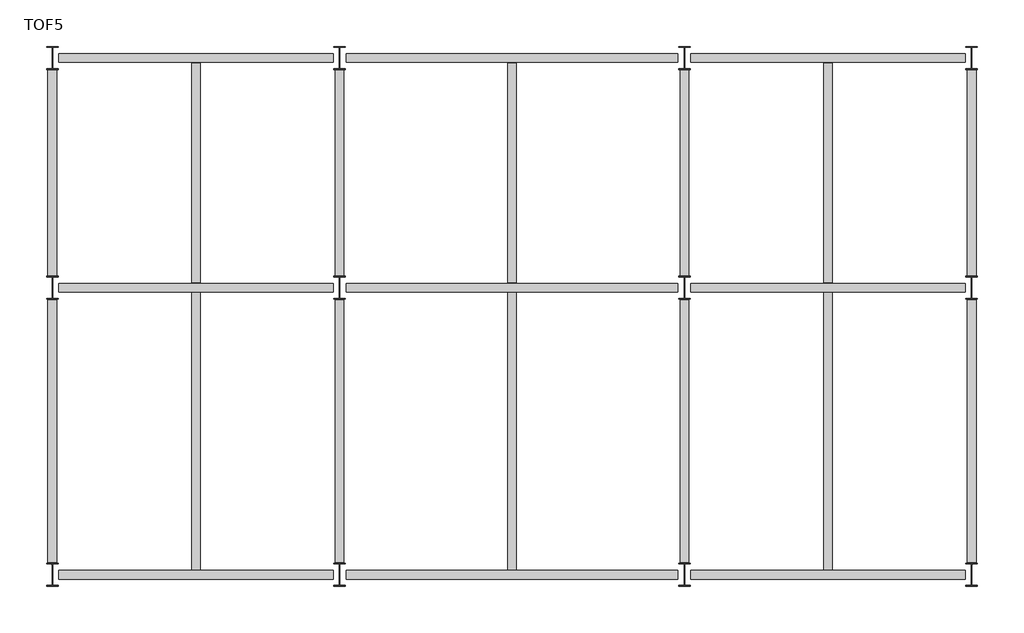
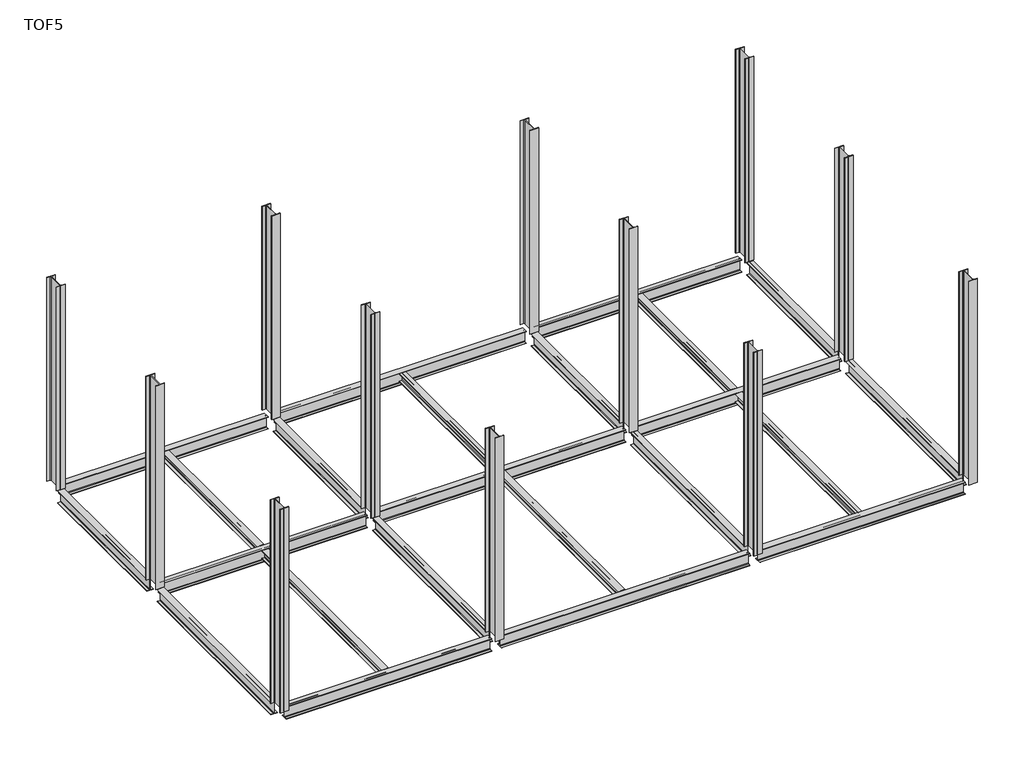
# One storey: 23 beams, 12 columns.
"""IFC4 building model written with IfcOpenShell, lengths in millimetres."""

import ifcopenshell
import ifcopenshell.guid

model = None  # the IFC model being written
_history = None  # IfcOwnerHistory: only IFC2X3 demands one
_inside = {}  # id of a spatial element -> (the spatial element, [elements in it])
_under = {}  # id of a project, library or spatial element -> (it, [spatial elements below it])
_declared = {}  # id of a project -> (the project, [libraries it declares])
_typed = {}  # id of a type object -> (the type object, [elements of that type])
_made_of = {}  # id of a material, layer set ... -> (it, [elements and type objects made of it])


def new_model(schema):
    """Start an empty IFC model of exactly this schema.

    Asked for "IFC4X3", IfcOpenShell would pick the latest addendum, in which some entities
    have other attributes; the version numbers below select the first issue.
    IFC2X3 requires an IfcOwnerHistory on every rooted entity: one is made here for all.
    """
    global model, _history
    if schema == "IFC4X3":
        model = ifcopenshell.file(schema_version=(4, 3, 0, 0))
    else:
        model = ifcopenshell.file(schema=schema)
    _inside.clear()
    _under.clear()
    _declared.clear()
    _typed.clear()
    _made_of.clear()
    _history = None
    if model.schema == "IFC2X3":
        org = make("IfcOrganization", Name="unknown")
        user = make(
            "IfcPersonAndOrganization",
            ThePerson=make("IfcPerson", FamilyName="unknown"),
            TheOrganization=org,
        )
        app = make(
            "IfcApplication",
            ApplicationDeveloper=org,
            Version="unknown",
            ApplicationFullName="unknown",
            ApplicationIdentifier="unknown",
        )
        _history = make(
            "IfcOwnerHistory",
            OwningUser=user,
            OwningApplication=app,
            ChangeAction="ADDED",
            CreationDate=0,
        )
    return model


def make(cls, **values):
    """One entity of the class cls with the attributes given. An attribute that is None is left unset."""
    return model.create_entity(
        cls, **{name: value for name, value in values.items() if value is not None}
    )


def rooted(cls, **values):
    """An entity with a GlobalId (a new one), such as an element, a storey or a relation."""
    return make(cls, GlobalId=ifcopenshell.guid.new(), OwnerHistory=_history, **values)


def si_unit(unit_type, name, prefix=None):
    """IfcSIUnit, for example si_unit("LENGTHUNIT", "METRE", prefix="MILLI")."""
    return make("IfcSIUnit", UnitType=unit_type, Prefix=prefix, Name=name)


def assignment(units):
    """IfcUnitAssignment: the units of a project."""
    return None if units is None else make("IfcUnitAssignment", Units=units)


def point(xyz):
    """IfcCartesianPoint."""
    return None if xyz is None else make("IfcCartesianPoint", Coordinates=xyz)


def direction(xyz):
    """IfcDirection."""
    return None if xyz is None else make("IfcDirection", DirectionRatios=xyz)


def frame(location, z_axis=None, x_axis=None):
    """IfcAxis2Placement3D, a coordinate frame: its origin and axes. An axis left out is left unset."""
    return make(
        "IfcAxis2Placement3D",
        Location=point(location),
        Axis=direction(z_axis),
        RefDirection=direction(x_axis),
    )


def frame_2d(location, x_axis=None):
    """IfcAxis2Placement2D, a coordinate frame in the plane: its origin and x axis."""
    return make(
        "IfcAxis2Placement2D", Location=point(location), RefDirection=direction(x_axis)
    )


def origin():
    """The frame at (0, 0, 0) with its axes left unset."""
    return frame((0.0, 0.0, 0.0))


def place(relative_to, where):
    """IfcLocalPlacement: puts the frame where relative to a parent placement (None: the world)."""
    return make(
        "IfcLocalPlacement", PlacementRelTo=relative_to, RelativePlacement=where
    )


def context(
    kind, dimensions, precision=None, world=None, true_north=None, identifier=None
):
    """IfcGeometricRepresentationContext, for example the 3D "Model" context."""
    return make(
        "IfcGeometricRepresentationContext",
        ContextIdentifier=identifier,
        ContextType=kind,
        CoordinateSpaceDimension=dimensions,
        Precision=precision,
        WorldCoordinateSystem=world,
        TrueNorth=true_north,
    )


def project(units=None, contexts=None):
    """IfcProject with its units and contexts."""
    return rooted(
        "IfcProject",
        Name="project",
        RepresentationContexts=contexts,
        UnitsInContext=assignment(units),
    )


def spatial(cls, under=None, at=None, **own):
    """A site, building, storey or space (cls), placed at a placement, below another one or the project."""
    s = rooted(cls, ObjectPlacement=at, **own)
    if under is not None:
        _under.setdefault(under.id(), (under, []))[1].append(s)
    return s


def polyline(points):
    """IfcPolyline through the points."""
    return make("IfcPolyline", Points=[point(p) for p in points])


def circle_curve(where, radius):
    """IfcCircle in the frame where."""
    return make("IfcCircle", Position=where, Radius=radius)


def trimmed(basis, trim1, trim2, sense, master):
    """IfcTrimmedCurve: the piece of a basis curve between two trims."""
    return make(
        "IfcTrimmedCurve",
        BasisCurve=basis,
        Trim1=trim1,
        Trim2=trim2,
        SenseAgreement=sense,
        MasterRepresentation=master,
    )


def segment(curve, same_sense, transition):
    """IfcCompositeCurveSegment."""
    return make(
        "IfcCompositeCurveSegment",
        Transition=transition,
        SameSense=same_sense,
        ParentCurve=curve,
    )


def composite_curve(segments, self_intersect=None):
    """IfcCompositeCurve: segments joined end to end."""
    return make("IfcCompositeCurve", Segments=segments, SelfIntersect=self_intersect)


def outline(outer, holes=None, kind="AREA"):
    """IfcArbitraryClosedProfileDef: a profile drawn as a closed curve; with holes, ...WithVoids."""
    if holes is None:
        return make("IfcArbitraryClosedProfileDef", ProfileType=kind, OuterCurve=outer)
    return make(
        "IfcArbitraryProfileDefWithVoids",
        ProfileType=kind,
        OuterCurve=outer,
        InnerCurves=holes,
    )


def extrude(swept, where, along, depth):
    """IfcExtrudedAreaSolid: the profile swept, set in the frame where, extruded along a direction by depth."""
    return make(
        "IfcExtrudedAreaSolid",
        SweptArea=swept,
        Position=where,
        ExtrudedDirection=direction(along),
        Depth=depth,
    )


def shape(context_of_items, identifier, shape_type, items):
    """IfcShapeRepresentation: the items that make up one representation, for example the "Body"."""
    return make(
        "IfcShapeRepresentation",
        ContextOfItems=context_of_items,
        RepresentationIdentifier=identifier,
        RepresentationType=shape_type,
        Items=items,
    )


def source(mapping_origin, context_of_items, identifier, shape_type, items):
    """IfcRepresentationMap: a shape defined once, which mapped items show again and again."""
    return make(
        "IfcRepresentationMap",
        MappingOrigin=mapping_origin,
        MappedRepresentation=shape(context_of_items, identifier, shape_type, items),
    )


def transform(
    local_origin,
    x_axis=None,
    y_axis=None,
    z_axis=None,
    scale=None,
    scale2=None,
    scale3=None,
    uniform=True,
):
    """IfcCartesianTransformationOperator3D, or its non-uniform kind. x_axis, y_axis, z_axis: its Axis1, 2, 3."""
    if uniform:
        return make(
            "IfcCartesianTransformationOperator3D",
            Axis1=direction(x_axis),
            Axis2=direction(y_axis),
            LocalOrigin=point(local_origin),
            Scale=scale,
            Axis3=direction(z_axis),
        )
    return make(
        "IfcCartesianTransformationOperator3DnonUniform",
        Axis1=direction(x_axis),
        Axis2=direction(y_axis),
        LocalOrigin=point(local_origin),
        Scale=scale,
        Axis3=direction(z_axis),
        Scale2=scale2,
        Scale3=scale3,
    )


def mapped(mapping_source, mapping_target):
    """IfcMappedItem: shows the shape of a source again, moved by a transform."""
    return make(
        "IfcMappedItem", MappingSource=mapping_source, MappingTarget=mapping_target
    )


def made_of(thing, what):
    """Note that an element or type object is made of a material, layer set ...; save() writes the relation."""
    if what is not None:
        _made_of.setdefault(what.id(), (what, []))[1].append(thing)
    return thing


def element(
    cls,
    number,
    at=None,
    inside=None,
    cuts=None,
    type_object=None,
    material=None,
    context=None,
    identifier="Body",
    shape_type=None,
    held_by="IfcProductDefinitionShape",
    body=None,
    shapes=None,
    **own,
):
    """One element of the class cls, such as IfcWall. Its Tag is "e" and its number.

    at: its placement. inside: the storey or other place that contains it. cuts: it is an
    opening in that element (IfcRelVoidsElement). A single representation is given by context,
    identifier, shape_type and body (its items); several are given by shapes. held_by: the class
    of the entity that holds the representations. save() writes the other relations.
    """
    e = rooted(cls, Tag="e%d" % number, ObjectPlacement=at, **own)
    if body is not None:
        shapes = [shape(context, identifier, shape_type, body)]
    if shapes is not None:
        e.Representation = make(held_by, Representations=shapes)
    if inside is not None:
        _inside.setdefault(inside.id(), (inside, []))[1].append(e)
    if cuts is not None:
        rooted(
            "IfcRelVoidsElement", RelatingBuildingElement=cuts, RelatedOpeningElement=e
        )
    if type_object is not None:
        _typed.setdefault(type_object.id(), (type_object, []))[1].append(e)
    return made_of(e, material)


def aggregate(whole, parts):
    """IfcRelAggregates: a whole, such as a stair, and the parts it consists of."""
    return rooted("IfcRelAggregates", RelatingObject=whole, RelatedObjects=parts)


def save(model, path):
    """Write the relations noted so far, then the file.

    IfcRelAggregates (storeys below a building ...), IfcRelContainedInSpatialStructure (elements
    in a storey), IfcRelDefinesByType, IfcRelAssociatesMaterial and IfcRelDeclares: one each for
    every whole, place, type object, material and project.
    """
    for whole, parts in _under.values():
        aggregate(whole, parts)
    for where, things in _inside.values():
        rooted(
            "IfcRelContainedInSpatialStructure",
            RelatedElements=things,
            RelatingStructure=where,
        )
    for kind, things in _typed.values():
        rooted("IfcRelDefinesByType", RelatedObjects=things, RelatingType=kind)
    for what, things in _made_of.values():
        rooted("IfcRelAssociatesMaterial", RelatedObjects=things, RelatingMaterial=what)
    for by, libraries in _declared.values():
        rooted("IfcRelDeclares", RelatingContext=by, RelatedDefinitions=libraries)
    model.write(path)


def beam_a4a24592(model_context):
    return source(origin(), model_context, "Body", "SweptSolid", [
        extrude(outline(composite_curve([segment(polyline([(75.0, -141.0), (75.0, -150.0), (-75.0, -150.0), (-75.0, -141.0), (-16.25, -141.0)]), True, "CONTINUOUS"), segment(trimmed(circle_curve(frame_2d((-16.25, -128.0)), 13.0), [point((-16.25, -141.0))], [point((-3.25, -128.0))], True, "CARTESIAN"), True, "CONTINUOUS"), segment(polyline([(-3.25, -128.0), (-3.25, 128.0)]), True, "CONTINUOUS"), segment(trimmed(circle_curve(frame_2d((-16.25, 128.0)), 13.0), [point((-3.25, 128.0))], [point((-16.25, 141.0))], True, "CARTESIAN"), True, "CONTINUOUS"), segment(polyline([(-16.25, 141.0), (-75.0, 141.0), (-75.0, 150.0), (75.0, 150.0), (75.0, 141.0), (16.25, 141.0)]), True, "CONTINUOUS"), segment(trimmed(circle_curve(frame_2d((16.25, 128.0)), 13.0), [point((16.25, 141.0))], [point((3.25, 128.0))], True, "CARTESIAN"), True, "CONTINUOUS"), segment(polyline([(3.25, 128.0), (3.25, -128.0)]), True, "CONTINUOUS"), segment(trimmed(circle_curve(frame_2d((16.25, -128.0)), 13.0), [point((3.25, -128.0))], [point((16.25, -141.0))], True, "CARTESIAN"), True, "CONTINUOUS"), segment(polyline([(16.25, -141.0), (75.0, -141.0)]), True, "CONTINUOUS")], self_intersect=False)), frame((-2387.3, 0.0, 0.0), z_axis=(1.0, 0.0, 0.0), x_axis=(0.0, 1.0, 0.0)), (0.0, 0.0, 1.0), 4774.6),
    ])


def beam_98be4253(model_context):
    return source(origin(), model_context, "Body", "SweptSolid", [
        extrude(outline(composite_curve([segment(polyline([(75.0, -141.0), (75.0, -150.0), (-75.0, -150.0), (-75.0, -141.0), (-16.25, -141.0)]), True, "CONTINUOUS"), segment(trimmed(circle_curve(frame_2d((-16.25, -128.0)), 13.0), [point((-16.25, -141.0))], [point((-3.25, -128.0))], True, "CARTESIAN"), True, "CONTINUOUS"), segment(polyline([(-3.25, -128.0), (-3.25, 128.0)]), True, "CONTINUOUS"), segment(trimmed(circle_curve(frame_2d((-16.25, 128.0)), 13.0), [point((-3.25, 128.0))], [point((-16.25, 141.0))], True, "CARTESIAN"), True, "CONTINUOUS"), segment(polyline([(-16.25, 141.0), (-75.0, 141.0), (-75.0, 150.0), (75.0, 150.0), (75.0, 141.0), (16.25, 141.0)]), True, "CONTINUOUS"), segment(trimmed(circle_curve(frame_2d((16.25, 128.0)), 13.0), [point((16.25, 141.0))], [point((3.25, 128.0))], True, "CARTESIAN"), True, "CONTINUOUS"), segment(polyline([(3.25, 128.0), (3.25, -128.0)]), True, "CONTINUOUS"), segment(trimmed(circle_curve(frame_2d((16.25, -128.0)), 13.0), [point((3.25, -128.0))], [point((16.25, -141.0))], True, "CARTESIAN"), True, "CONTINUOUS"), segment(polyline([(16.25, -141.0), (75.0, -141.0)]), True, "CONTINUOUS")], self_intersect=False)), frame((-2887.3, 0.0, 0.0), z_axis=(1.0, 0.0, 0.0), x_axis=(0.0, 1.0, 0.0)), (0.0, 0.0, 1.0), 5774.6),
    ])


def beam_4b5297f3(model_context):
    return source(origin(), model_context, "Body", "SweptSolid", [
        extrude(outline(composite_curve([segment(polyline([(75.0, -141.0), (75.0, -150.0), (-75.0, -150.0), (-75.0, -141.0), (-16.25, -141.0)]), True, "CONTINUOUS"), segment(trimmed(circle_curve(frame_2d((-16.25, -128.0)), 13.0), [point((-16.25, -141.0))], [point((-3.25, -128.0))], True, "CARTESIAN"), True, "CONTINUOUS"), segment(polyline([(-3.25, -128.0), (-3.25, 128.0)]), True, "CONTINUOUS"), segment(trimmed(circle_curve(frame_2d((-16.25, 128.0)), 13.0), [point((-3.25, 128.0))], [point((-16.25, 141.0))], True, "CARTESIAN"), True, "CONTINUOUS"), segment(polyline([(-16.25, 141.0), (-75.0, 141.0), (-75.0, 150.0), (75.0, 150.0), (75.0, 141.0), (16.25, 141.0)]), True, "CONTINUOUS"), segment(trimmed(circle_curve(frame_2d((16.25, 128.0)), 13.0), [point((16.25, 141.0))], [point((3.25, 128.0))], True, "CARTESIAN"), True, "CONTINUOUS"), segment(polyline([(3.25, 128.0), (3.25, -128.0)]), True, "CONTINUOUS"), segment(trimmed(circle_curve(frame_2d((16.25, -128.0)), 13.0), [point((3.25, -128.0))], [point((16.25, -141.0))], True, "CARTESIAN"), True, "CONTINUOUS"), segment(polyline([(16.25, -141.0), (75.0, -141.0)]), True, "CONTINUOUS")], self_intersect=False)), frame((-2287.3, 0.0, 0.0), z_axis=(1.0, 0.0, 0.0), x_axis=(0.0, 1.0, 0.0)), (0.0, 0.0, 1.0), 4574.6),
    ])


def beam_dad7a266(model_context):
    return source(origin(), model_context, "Body", "SweptSolid", [
        extrude(outline(composite_curve([segment(polyline([(75.0, -141.0), (75.0, -150.0), (-75.0, -150.0), (-75.0, -141.0), (-16.25, -141.0)]), True, "CONTINUOUS"), segment(trimmed(circle_curve(frame_2d((-16.25, -128.0)), 13.0), [point((-16.25, -141.0))], [point((-3.25, -128.0))], True, "CARTESIAN"), True, "CONTINUOUS"), segment(polyline([(-3.25, -128.0), (-3.25, 128.0)]), True, "CONTINUOUS"), segment(trimmed(circle_curve(frame_2d((-16.25, 128.0)), 13.0), [point((-3.25, 128.0))], [point((-16.25, 141.0))], True, "CARTESIAN"), True, "CONTINUOUS"), segment(polyline([(-16.25, 141.0), (-75.0, 141.0), (-75.0, 150.0), (75.0, 150.0), (75.0, 141.0), (16.25, 141.0)]), True, "CONTINUOUS"), segment(trimmed(circle_curve(frame_2d((16.25, 128.0)), 13.0), [point((16.25, 141.0))], [point((3.25, 128.0))], True, "CARTESIAN"), True, "CONTINUOUS"), segment(polyline([(3.25, 128.0), (3.25, -128.0)]), True, "CONTINUOUS"), segment(trimmed(circle_curve(frame_2d((16.25, -128.0)), 13.0), [point((3.25, -128.0))], [point((16.25, -141.0))], True, "CARTESIAN"), True, "CONTINUOUS"), segment(polyline([(16.25, -141.0), (75.0, -141.0)]), True, "CONTINUOUS")], self_intersect=False)), frame((-1787.3, 0.0, 0.0), z_axis=(1.0, 0.0, 0.0), x_axis=(0.0, 1.0, 0.0)), (0.0, 0.0, 1.0), 3574.6),
    ])


def beam_719db1ac(model_context):
    return source(origin(), model_context, "Body", "SweptSolid", [
        extrude(outline(composite_curve([segment(polyline([(75.0, -88.0), (75.0, -97.0), (-75.0, -97.0), (-75.0, -88.0), (-16.0, -88.0)]), True, "CONTINUOUS"), segment(trimmed(circle_curve(frame_2d((-16.0, -75.0)), 13.0), [point((-16.0, -88.0))], [point((-3.0, -75.0))], True, "CARTESIAN"), True, "CONTINUOUS"), segment(polyline([(-3.0, -75.0), (-3.0, 75.0)]), True, "CONTINUOUS"), segment(trimmed(circle_curve(frame_2d((-16.0, 75.0)), 13.0), [point((-3.0, 75.0))], [point((-16.0, 88.0))], True, "CARTESIAN"), True, "CONTINUOUS"), segment(polyline([(-16.0, 88.0), (-75.0, 88.0), (-75.0, 97.0), (75.0, 97.0), (75.0, 88.0), (16.0, 88.0)]), True, "CONTINUOUS"), segment(trimmed(circle_curve(frame_2d((16.0, 75.0)), 13.0), [point((16.0, 88.0))], [point((3.0, 75.0))], True, "CARTESIAN"), True, "CONTINUOUS"), segment(polyline([(3.0, 75.0), (3.0, -75.0)]), True, "CONTINUOUS"), segment(trimmed(circle_curve(frame_2d((16.0, -75.0)), 13.0), [point((3.0, -75.0))], [point((16.0, -88.0))], True, "CARTESIAN"), True, "CONTINUOUS"), segment(polyline([(16.0, -88.0), (75.0, -88.0)]), True, "CONTINUOUS")], self_intersect=False)), frame((-2412.3, 0.0, 0.0), z_axis=(1.0, 0.0, 0.0), x_axis=(0.0, 1.0, 0.0)), (0.0, 0.0, 1.0), 4824.6),
    ])


def beam_533db150(model_context):
    return source(origin(), model_context, "Body", "SweptSolid", [
        extrude(outline(composite_curve([segment(polyline([(75.0, -88.0), (75.0, -97.0), (-75.0, -97.0), (-75.0, -88.0), (-16.0, -88.0)]), True, "CONTINUOUS"), segment(trimmed(circle_curve(frame_2d((-16.0, -75.0)), 13.0), [point((-16.0, -88.0))], [point((-3.0, -75.0))], True, "CARTESIAN"), True, "CONTINUOUS"), segment(polyline([(-3.0, -75.0), (-3.0, 75.0)]), True, "CONTINUOUS"), segment(trimmed(circle_curve(frame_2d((-16.0, 75.0)), 13.0), [point((-3.0, 75.0))], [point((-16.0, 88.0))], True, "CARTESIAN"), True, "CONTINUOUS"), segment(polyline([(-16.0, 88.0), (-75.0, 88.0), (-75.0, 97.0), (75.0, 97.0), (75.0, 88.0), (16.0, 88.0)]), True, "CONTINUOUS"), segment(trimmed(circle_curve(frame_2d((16.0, 75.0)), 13.0), [point((16.0, 88.0))], [point((3.0, 75.0))], True, "CARTESIAN"), True, "CONTINUOUS"), segment(polyline([(3.0, 75.0), (3.0, -75.0)]), True, "CONTINUOUS"), segment(trimmed(circle_curve(frame_2d((16.0, -75.0)), 13.0), [point((3.0, -75.0))], [point((16.0, -88.0))], True, "CARTESIAN"), True, "CONTINUOUS"), segment(polyline([(16.0, -88.0), (75.0, -88.0)]), True, "CONTINUOUS")], self_intersect=False)), frame((-1912.3, 0.0, 0.0), z_axis=(1.0, 0.0, 0.0), x_axis=(0.0, 1.0, 0.0)), (0.0, 0.0, 1.0), 3824.6),
    ])


model = new_model("IFC4")

# Units and contexts
model_context = context("Model", 3, world=origin())
ifc_project = project(units=[si_unit("LENGTHUNIT", "METRE", prefix="MILLI")], contexts=[model_context])

# Site, building, storey
site = spatial("IfcSite", under=ifc_project)
building = spatial("IfcBuilding", under=site)
storey = spatial("IfcBuildingStorey", under=building, Name="TOF5", Elevation=4000.0)

# Beams
placement = place(None, origin())
beam_shape = beam_a4a24592(model_context)
element("IfcBeam", 1, ObjectType="0912_Steel Framing_H-KSD3502 : H_SB_AR_S02_H-300x150x6.5x9_Stair", at=placement, inside=storey, context=model_context, shape_type="MappedRepresentation", body=[
    mapped(beam_shape, transform((2500.0, 0.0, 3850.0), x_axis=(1.0, 0.0, 0.0), y_axis=(0.0, 1.0, 0.0), z_axis=(0.0, 0.0, 1.0))),
])
element("IfcBeam", 2, ObjectType="0912_Steel Framing_H-KSD3502 : H_SB_AR_S02_H-300x150x6.5x9_Stair", at=placement, inside=storey, context=model_context, shape_type="MappedRepresentation", body=[
    mapped(beam_shape, transform((13500.0, 0.0, 3850.0), x_axis=(1.0, 0.0, 0.0), y_axis=(0.0, 1.0, 0.0), z_axis=(0.0, 0.0, 1.0))),
])
element("IfcBeam", 3, ObjectType="0912_Steel Framing_H-KSD3502 : H_SB_AR_S02_H-300x150x6.5x9_Stair", at=placement, inside=storey, context=model_context, shape_type="MappedRepresentation", body=[
    mapped(beam_shape, transform((2500.0, 5000.0, 3850.0), x_axis=(1.0, 0.0, 0.0), y_axis=(0.0, 1.0, 0.0), z_axis=(0.0, 0.0, 1.0))),
])
element("IfcBeam", 4, ObjectType="0912_Steel Framing_H-KSD3502 : H_SB_AR_S02_H-300x150x6.5x9_Stair", at=placement, inside=storey, context=model_context, shape_type="MappedRepresentation", body=[
    mapped(beam_shape, transform((13500.0, 5000.0, 3850.0), x_axis=(1.0, 0.0, 0.0), y_axis=(0.0, 1.0, 0.0), z_axis=(0.0, 0.0, 1.0))),
])
element("IfcBeam", 5, ObjectType="0912_Steel Framing_H-KSD3502 : H_SB_AR_S02_H-300x150x6.5x9_Stair", at=placement, inside=storey, context=model_context, shape_type="MappedRepresentation", body=[
    mapped(beam_shape, transform((2500.0, 9000.0, 3850.0), x_axis=(1.0, 0.0, 0.0), y_axis=(0.0, 1.0, 0.0), z_axis=(0.0, 0.0, 1.0))),
])
element("IfcBeam", 6, ObjectType="0912_Steel Framing_H-KSD3502 : H_SB_AR_S02_H-300x150x6.5x9_Stair", at=placement, inside=storey, context=model_context, shape_type="MappedRepresentation", body=[
    mapped(beam_shape, transform((13500.0, 9000.0, 3850.0), x_axis=(1.0, 0.0, 0.0), y_axis=(0.0, 1.0, 0.0), z_axis=(0.0, 0.0, 1.0))),
])
beam_2_shape = beam_98be4253(model_context)
element("IfcBeam", 7, ObjectType="0912_Steel Framing_H-KSD3502 : H_SB_AR_S02_H-300x150x6.5x9_Stair", at=placement, inside=storey, context=model_context, shape_type="MappedRepresentation", body=[
    mapped(beam_2_shape, transform((8000.0, 0.0, 3850.0), x_axis=(1.0, 0.0, 0.0), y_axis=(0.0, 1.0, 0.0), z_axis=(0.0, 0.0, 1.0))),
])
element("IfcBeam", 8, ObjectType="0912_Steel Framing_H-KSD3502 : H_SB_AR_S02_H-300x150x6.5x9_Stair", at=placement, inside=storey, context=model_context, shape_type="MappedRepresentation", body=[
    mapped(beam_2_shape, transform((8000.0, 5000.0, 3850.0), x_axis=(1.0, 0.0, 0.0), y_axis=(0.0, 1.0, 0.0), z_axis=(0.0, 0.0, 1.0))),
])
element("IfcBeam", 9, ObjectType="0912_Steel Framing_H-KSD3502 : H_SB_AR_S02_H-300x150x6.5x9_Stair", at=placement, inside=storey, context=model_context, shape_type="MappedRepresentation", body=[
    mapped(beam_2_shape, transform((8000.0, 9000.0, 3850.0), x_axis=(1.0, 0.0, 0.0), y_axis=(0.0, 1.0, 0.0), z_axis=(0.0, 0.0, 1.0))),
])
beam_3_shape = beam_4b5297f3(model_context)
element("IfcBeam", 10, ObjectType="0912_Steel Framing_H-KSD3502 : H_SB_AR_S02_H-300x150x6.5x9_Stair", at=placement, inside=storey, context=model_context, shape_type="MappedRepresentation", body=[
    mapped(beam_3_shape, transform((0.0, 2500.0, 3850.0), x_axis=(0.0, 1.0, 0.0), y_axis=(-1.0, 0.0, 0.0), z_axis=(0.0, 0.0, 1.0))),
])
element("IfcBeam", 11, ObjectType="0912_Steel Framing_H-KSD3502 : H_SB_AR_S02_H-300x150x6.5x9_Stair", at=placement, inside=storey, context=model_context, shape_type="MappedRepresentation", body=[
    mapped(beam_3_shape, transform((5000.0, 2500.0, 3850.0), x_axis=(0.0, 1.0, 0.0), y_axis=(-1.0, 0.0, 0.0), z_axis=(0.0, 0.0, 1.0))),
])
element("IfcBeam", 12, ObjectType="0912_Steel Framing_H-KSD3502 : H_SB_AR_S02_H-300x150x6.5x9_Stair", at=placement, inside=storey, context=model_context, shape_type="MappedRepresentation", body=[
    mapped(beam_3_shape, transform((11000.0, 2500.0, 3850.0), x_axis=(0.0, 1.0, 0.0), y_axis=(-1.0, 0.0, 0.0), z_axis=(0.0, 0.0, 1.0))),
])
element("IfcBeam", 13, ObjectType="0912_Steel Framing_H-KSD3502 : H_SB_AR_S02_H-300x150x6.5x9_Stair", at=placement, inside=storey, context=model_context, shape_type="MappedRepresentation", body=[
    mapped(beam_3_shape, transform((16000.0, 2500.0, 3850.0), x_axis=(0.0, 1.0, 0.0), y_axis=(-1.0, 0.0, 0.0), z_axis=(0.0, 0.0, 1.0))),
])
beam_4_shape = beam_dad7a266(model_context)
element("IfcBeam", 14, ObjectType="0912_Steel Framing_H-KSD3502 : H_SB_AR_S02_H-300x150x6.5x9_Stair", at=placement, inside=storey, context=model_context, shape_type="MappedRepresentation", body=[
    mapped(beam_4_shape, transform((0.0, 7000.0, 3850.0), x_axis=(0.0, 1.0, 0.0), y_axis=(-1.0, 0.0, 0.0), z_axis=(0.0, 0.0, 1.0))),
])
element("IfcBeam", 15, ObjectType="0912_Steel Framing_H-KSD3502 : H_SB_AR_S02_H-300x150x6.5x9_Stair", at=placement, inside=storey, context=model_context, shape_type="MappedRepresentation", body=[
    mapped(beam_4_shape, transform((5000.0, 7000.0, 3850.0), x_axis=(0.0, 1.0, 0.0), y_axis=(-1.0, 0.0, 0.0), z_axis=(0.0, 0.0, 1.0))),
])
element("IfcBeam", 16, ObjectType="0912_Steel Framing_H-KSD3502 : H_SB_AR_S02_H-300x150x6.5x9_Stair", at=placement, inside=storey, context=model_context, shape_type="MappedRepresentation", body=[
    mapped(beam_4_shape, transform((11000.0, 7000.0, 3850.0), x_axis=(0.0, 1.0, 0.0), y_axis=(-1.0, 0.0, 0.0), z_axis=(0.0, 0.0, 1.0))),
])
element("IfcBeam", 17, ObjectType="0912_Steel Framing_H-KSD3502 : H_SB_AR_S02_H-300x150x6.5x9_Stair", at=placement, inside=storey, context=model_context, shape_type="MappedRepresentation", body=[
    mapped(beam_4_shape, transform((16000.0, 7000.0, 3850.0), x_axis=(0.0, 1.0, 0.0), y_axis=(-1.0, 0.0, 0.0), z_axis=(0.0, 0.0, 1.0))),
])
beam_5_shape = beam_719db1ac(model_context)
element("IfcBeam", 18, ObjectType="0912_Steel Framing_H-KSD3502 : H_SB_AR_S02_H-194x150x6x9_Platform", at=placement, inside=storey, context=model_context, shape_type="MappedRepresentation", body=[
    mapped(beam_5_shape, transform((2500.0, 2500.0, 3903.0), x_axis=(0.0, 1.0, 0.0), y_axis=(-1.0, 0.0, 0.0), z_axis=(0.0, 0.0, 1.0))),
])
element("IfcBeam", 19, ObjectType="0912_Steel Framing_H-KSD3502 : H_SB_AR_S02_H-194x150x6x9_Platform", at=placement, inside=storey, context=model_context, shape_type="MappedRepresentation", body=[
    mapped(beam_5_shape, transform((8000.0, 2500.0, 3903.0), x_axis=(0.0, 1.0, 0.0), y_axis=(-1.0, 0.0, 0.0), z_axis=(0.0, 0.0, 1.0))),
])
element("IfcBeam", 20, ObjectType="0912_Steel Framing_H-KSD3502 : H_SB_AR_S02_H-194x150x6x9_Platform", at=placement, inside=storey, context=model_context, shape_type="MappedRepresentation", body=[
    mapped(beam_5_shape, transform((13500.0, 2500.0, 3903.0), x_axis=(0.0, 1.0, 0.0), y_axis=(-1.0, 0.0, 0.0), z_axis=(0.0, 0.0, 1.0))),
])
beam_6_shape = beam_533db150(model_context)
element("IfcBeam", 21, ObjectType="0912_Steel Framing_H-KSD3502 : H_SB_AR_S02_H-194x150x6x9_Platform", at=placement, inside=storey, context=model_context, shape_type="MappedRepresentation", body=[
    mapped(beam_6_shape, transform((2500.0, 7000.0, 3903.0), x_axis=(0.0, 1.0, 0.0), y_axis=(-1.0, 0.0, 0.0), z_axis=(0.0, 0.0, 1.0))),
])
element("IfcBeam", 22, ObjectType="0912_Steel Framing_H-KSD3502 : H_SB_AR_S02_H-194x150x6x9_Platform", at=placement, inside=storey, context=model_context, shape_type="MappedRepresentation", body=[
    mapped(beam_6_shape, transform((8000.0, 7000.0, 3903.0), x_axis=(0.0, 1.0, 0.0), y_axis=(-1.0, 0.0, 0.0), z_axis=(0.0, 0.0, 1.0))),
])
element("IfcBeam", 23, ObjectType="0912_Steel Framing_H-KSD3502 : H_SB_AR_S02_H-194x150x6x9_Platform", at=placement, inside=storey, context=model_context, shape_type="MappedRepresentation", body=[
    mapped(beam_6_shape, transform((13500.0, 7000.0, 3903.0), x_axis=(0.0, 1.0, 0.0), y_axis=(-1.0, 0.0, 0.0), z_axis=(0.0, 0.0, 1.0))),
])

# Columns
element("IfcColumn", 24, ObjectType="Steel Column_H_KSD3502 : H_SC_AR_S01_H-400x200x8x13", at=placement, inside=storey, context=model_context, shape_type="SweptSolid", body=[
    extrude(outline(composite_curve([segment(polyline([(100.0, 200.0), (100.0, 187.0), (20.0, 187.0)]), True, "CONTINUOUS"), segment(trimmed(circle_curve(frame_2d((20.0, 171.0)), 16.0), [point((20.0, 187.0))], [point((4.0, 171.0))], True, "CARTESIAN"), True, "CONTINUOUS"), segment(polyline([(4.0, 171.0), (4.0, -171.0)]), True, "CONTINUOUS"), segment(trimmed(circle_curve(frame_2d((20.0, -171.0)), 16.0), [point((4.0, -171.0))], [point((20.0, -187.0))], True, "CARTESIAN"), True, "CONTINUOUS"), segment(polyline([(20.0, -187.0), (100.0, -187.0), (100.0, -200.0), (-100.0, -200.0), (-100.0, -187.0), (-20.0, -187.0)]), True, "CONTINUOUS"), segment(trimmed(circle_curve(frame_2d((-20.0, -171.0)), 16.0), [point((-20.0, -187.0))], [point((-4.0, -171.0))], True, "CARTESIAN"), True, "CONTINUOUS"), segment(polyline([(-4.0, -171.0), (-4.0, 171.0)]), True, "CONTINUOUS"), segment(trimmed(circle_curve(frame_2d((-20.0, 171.0)), 16.0), [point((-4.0, 171.0))], [point((-20.0, 187.0))], True, "CARTESIAN"), True, "CONTINUOUS"), segment(polyline([(-20.0, 187.0), (-100.0, 187.0), (-100.0, 200.0), (100.0, 200.0)]), True, "CONTINUOUS")], self_intersect=False)), frame((0.0, 0.0, 4000.0), z_axis=(0.0, 0.0, 1.0), x_axis=(1.0, 0.0, 0.0)), (0.0, 0.0, 1.0), 5000.0),
])
element("IfcColumn", 25, ObjectType="Steel Column_H_KSD3502 : H_SC_AR_S01_H-400x200x8x13", at=placement, inside=storey, context=model_context, shape_type="SweptSolid", body=[
    extrude(outline(composite_curve([segment(polyline([(5100.0, 200.0), (5100.0, 187.0), (5020.0, 187.0)]), True, "CONTINUOUS"), segment(trimmed(circle_curve(frame_2d((5020.0, 171.0)), 16.0), [point((5020.0, 187.0))], [point((5004.0, 171.0))], True, "CARTESIAN"), True, "CONTINUOUS"), segment(polyline([(5004.0, 171.0), (5004.0, -171.0)]), True, "CONTINUOUS"), segment(trimmed(circle_curve(frame_2d((5020.0, -171.0)), 16.0), [point((5004.0, -171.0))], [point((5020.0, -187.0))], True, "CARTESIAN"), True, "CONTINUOUS"), segment(polyline([(5020.0, -187.0), (5100.0, -187.0), (5100.0, -200.0), (4900.0, -200.0), (4900.0, -187.0), (4980.0, -187.0)]), True, "CONTINUOUS"), segment(trimmed(circle_curve(frame_2d((4980.0, -171.0)), 16.0), [point((4980.0, -187.0))], [point((4996.0, -171.0))], True, "CARTESIAN"), True, "CONTINUOUS"), segment(polyline([(4996.0, -171.0), (4996.0, 171.0)]), True, "CONTINUOUS"), segment(trimmed(circle_curve(frame_2d((4980.0, 171.0)), 16.0), [point((4996.0, 171.0))], [point((4980.0, 187.0))], True, "CARTESIAN"), True, "CONTINUOUS"), segment(polyline([(4980.0, 187.0), (4900.0, 187.0), (4900.0, 200.0), (5100.0, 200.0)]), True, "CONTINUOUS")], self_intersect=False)), frame((0.0, 0.0, 4000.0), z_axis=(0.0, 0.0, 1.0), x_axis=(1.0, 0.0, 0.0)), (0.0, 0.0, 1.0), 5000.0),
])
element("IfcColumn", 26, ObjectType="Steel Column_H_KSD3502 : H_SC_AR_S01_H-400x200x8x13", at=placement, inside=storey, context=model_context, shape_type="SweptSolid", body=[
    extrude(outline(composite_curve([segment(polyline([(11100.0, 200.0), (11100.0, 187.0), (11020.0, 187.0)]), True, "CONTINUOUS"), segment(trimmed(circle_curve(frame_2d((11020.0, 171.0)), 16.0), [point((11020.0, 187.0))], [point((11004.0, 171.0))], True, "CARTESIAN"), True, "CONTINUOUS"), segment(polyline([(11004.0, 171.0), (11004.0, -171.0)]), True, "CONTINUOUS"), segment(trimmed(circle_curve(frame_2d((11020.0, -171.0)), 16.0), [point((11004.0, -171.0))], [point((11020.0, -187.0))], True, "CARTESIAN"), True, "CONTINUOUS"), segment(polyline([(11020.0, -187.0), (11100.0, -187.0), (11100.0, -200.0), (10900.0, -200.0), (10900.0, -187.0), (10980.0, -187.0)]), True, "CONTINUOUS"), segment(trimmed(circle_curve(frame_2d((10980.0, -171.0)), 16.0), [point((10980.0, -187.0))], [point((10996.0, -171.0))], True, "CARTESIAN"), True, "CONTINUOUS"), segment(polyline([(10996.0, -171.0), (10996.0, 171.0)]), True, "CONTINUOUS"), segment(trimmed(circle_curve(frame_2d((10980.0, 171.0)), 16.0), [point((10996.0, 171.0))], [point((10980.0, 187.0))], True, "CARTESIAN"), True, "CONTINUOUS"), segment(polyline([(10980.0, 187.0), (10900.0, 187.0), (10900.0, 200.0), (11100.0, 200.0)]), True, "CONTINUOUS")], self_intersect=False)), frame((0.0, 0.0, 4000.0), z_axis=(0.0, 0.0, 1.0), x_axis=(1.0, 0.0, 0.0)), (0.0, 0.0, 1.0), 5000.0),
])
element("IfcColumn", 27, ObjectType="Steel Column_H_KSD3502 : H_SC_AR_S01_H-400x200x8x13", at=placement, inside=storey, context=model_context, shape_type="SweptSolid", body=[
    extrude(outline(composite_curve([segment(polyline([(16100.0, 200.0), (16100.0, 187.0), (16020.0, 187.0)]), True, "CONTINUOUS"), segment(trimmed(circle_curve(frame_2d((16020.0, 171.0)), 16.0), [point((16020.0, 187.0))], [point((16004.0, 171.0))], True, "CARTESIAN"), True, "CONTINUOUS"), segment(polyline([(16004.0, 171.0), (16004.0, -171.0)]), True, "CONTINUOUS"), segment(trimmed(circle_curve(frame_2d((16020.0, -171.0)), 16.0), [point((16004.0, -171.0))], [point((16020.0, -187.0))], True, "CARTESIAN"), True, "CONTINUOUS"), segment(polyline([(16020.0, -187.0), (16100.0, -187.0), (16100.0, -200.0), (15900.0, -200.0), (15900.0, -187.0), (15980.0, -187.0)]), True, "CONTINUOUS"), segment(trimmed(circle_curve(frame_2d((15980.0, -171.0)), 16.0), [point((15980.0, -187.0))], [point((15996.0, -171.0))], True, "CARTESIAN"), True, "CONTINUOUS"), segment(polyline([(15996.0, -171.0), (15996.0, 171.0)]), True, "CONTINUOUS"), segment(trimmed(circle_curve(frame_2d((15980.0, 171.0)), 16.0), [point((15996.0, 171.0))], [point((15980.0, 187.0))], True, "CARTESIAN"), True, "CONTINUOUS"), segment(polyline([(15980.0, 187.0), (15900.0, 187.0), (15900.0, 200.0), (16100.0, 200.0)]), True, "CONTINUOUS")], self_intersect=False)), frame((0.0, 0.0, 4000.0), z_axis=(0.0, 0.0, 1.0), x_axis=(1.0, 0.0, 0.0)), (0.0, 0.0, 1.0), 5000.0),
])
element("IfcColumn", 28, ObjectType="Steel Column_H_KSD3502 : H_SC_AR_S01_H-400x200x8x13", at=placement, inside=storey, context=model_context, shape_type="SweptSolid", body=[
    extrude(outline(composite_curve([segment(polyline([(100.0, 5200.0), (100.0, 5187.0), (20.0, 5187.0)]), True, "CONTINUOUS"), segment(trimmed(circle_curve(frame_2d((20.0, 5171.0)), 16.0), [point((20.0, 5187.0))], [point((4.0, 5171.0))], True, "CARTESIAN"), True, "CONTINUOUS"), segment(polyline([(4.0, 5171.0), (4.0, 4829.0)]), True, "CONTINUOUS"), segment(trimmed(circle_curve(frame_2d((20.0, 4829.0)), 16.0), [point((4.0, 4829.0))], [point((20.0, 4813.0))], True, "CARTESIAN"), True, "CONTINUOUS"), segment(polyline([(20.0, 4813.0), (100.0, 4813.0), (100.0, 4800.0), (-100.0, 4800.0), (-100.0, 4813.0), (-20.0, 4813.0)]), True, "CONTINUOUS"), segment(trimmed(circle_curve(frame_2d((-20.0, 4829.0)), 16.0), [point((-20.0, 4813.0))], [point((-4.0, 4829.0))], True, "CARTESIAN"), True, "CONTINUOUS"), segment(polyline([(-4.0, 4829.0), (-4.0, 5171.0)]), True, "CONTINUOUS"), segment(trimmed(circle_curve(frame_2d((-20.0, 5171.0)), 16.0), [point((-4.0, 5171.0))], [point((-20.0, 5187.0))], True, "CARTESIAN"), True, "CONTINUOUS"), segment(polyline([(-20.0, 5187.0), (-100.0, 5187.0), (-100.0, 5200.0), (100.0, 5200.0)]), True, "CONTINUOUS")], self_intersect=False)), frame((0.0, 0.0, 4000.0), z_axis=(0.0, 0.0, 1.0), x_axis=(1.0, 0.0, 0.0)), (0.0, 0.0, 1.0), 5000.0),
])
element("IfcColumn", 29, ObjectType="Steel Column_H_KSD3502 : H_SC_AR_S01_H-400x200x8x13", at=placement, inside=storey, context=model_context, shape_type="SweptSolid", body=[
    extrude(outline(composite_curve([segment(polyline([(5100.0, 5200.0), (5100.0, 5187.0), (5020.0, 5187.0)]), True, "CONTINUOUS"), segment(trimmed(circle_curve(frame_2d((5020.0, 5171.0)), 16.0), [point((5020.0, 5187.0))], [point((5004.0, 5171.0))], True, "CARTESIAN"), True, "CONTINUOUS"), segment(polyline([(5004.0, 5171.0), (5004.0, 4829.0)]), True, "CONTINUOUS"), segment(trimmed(circle_curve(frame_2d((5020.0, 4829.0)), 16.0), [point((5004.0, 4829.0))], [point((5020.0, 4813.0))], True, "CARTESIAN"), True, "CONTINUOUS"), segment(polyline([(5020.0, 4813.0), (5100.0, 4813.0), (5100.0, 4800.0), (4900.0, 4800.0), (4900.0, 4813.0), (4980.0, 4813.0)]), True, "CONTINUOUS"), segment(trimmed(circle_curve(frame_2d((4980.0, 4829.0)), 16.0), [point((4980.0, 4813.0))], [point((4996.0, 4829.0))], True, "CARTESIAN"), True, "CONTINUOUS"), segment(polyline([(4996.0, 4829.0), (4996.0, 5171.0)]), True, "CONTINUOUS"), segment(trimmed(circle_curve(frame_2d((4980.0, 5171.0)), 16.0), [point((4996.0, 5171.0))], [point((4980.0, 5187.0))], True, "CARTESIAN"), True, "CONTINUOUS"), segment(polyline([(4980.0, 5187.0), (4900.0, 5187.0), (4900.0, 5200.0), (5100.0, 5200.0)]), True, "CONTINUOUS")], self_intersect=False)), frame((0.0, 0.0, 4000.0), z_axis=(0.0, 0.0, 1.0), x_axis=(1.0, 0.0, 0.0)), (0.0, 0.0, 1.0), 5000.0),
])
element("IfcColumn", 30, ObjectType="Steel Column_H_KSD3502 : H_SC_AR_S01_H-400x200x8x13", at=placement, inside=storey, context=model_context, shape_type="SweptSolid", body=[
    extrude(outline(composite_curve([segment(polyline([(11100.0, 5200.0), (11100.0, 5187.0), (11020.0, 5187.0)]), True, "CONTINUOUS"), segment(trimmed(circle_curve(frame_2d((11020.0, 5171.0)), 16.0), [point((11020.0, 5187.0))], [point((11004.0, 5171.0))], True, "CARTESIAN"), True, "CONTINUOUS"), segment(polyline([(11004.0, 5171.0), (11004.0, 4829.0)]), True, "CONTINUOUS"), segment(trimmed(circle_curve(frame_2d((11020.0, 4829.0)), 16.0), [point((11004.0, 4829.0))], [point((11020.0, 4813.0))], True, "CARTESIAN"), True, "CONTINUOUS"), segment(polyline([(11020.0, 4813.0), (11100.0, 4813.0), (11100.0, 4800.0), (10900.0, 4800.0), (10900.0, 4813.0), (10980.0, 4813.0)]), True, "CONTINUOUS"), segment(trimmed(circle_curve(frame_2d((10980.0, 4829.0)), 16.0), [point((10980.0, 4813.0))], [point((10996.0, 4829.0))], True, "CARTESIAN"), True, "CONTINUOUS"), segment(polyline([(10996.0, 4829.0), (10996.0, 5171.0)]), True, "CONTINUOUS"), segment(trimmed(circle_curve(frame_2d((10980.0, 5171.0)), 16.0), [point((10996.0, 5171.0))], [point((10980.0, 5187.0))], True, "CARTESIAN"), True, "CONTINUOUS"), segment(polyline([(10980.0, 5187.0), (10900.0, 5187.0), (10900.0, 5200.0), (11100.0, 5200.0)]), True, "CONTINUOUS")], self_intersect=False)), frame((0.0, 0.0, 4000.0), z_axis=(0.0, 0.0, 1.0), x_axis=(1.0, 0.0, 0.0)), (0.0, 0.0, 1.0), 5000.0),
])
element("IfcColumn", 31, ObjectType="Steel Column_H_KSD3502 : H_SC_AR_S01_H-400x200x8x13", at=placement, inside=storey, context=model_context, shape_type="SweptSolid", body=[
    extrude(outline(composite_curve([segment(polyline([(16100.0, 5200.0), (16100.0, 5187.0), (16020.0, 5187.0)]), True, "CONTINUOUS"), segment(trimmed(circle_curve(frame_2d((16020.0, 5171.0)), 16.0), [point((16020.0, 5187.0))], [point((16004.0, 5171.0))], True, "CARTESIAN"), True, "CONTINUOUS"), segment(polyline([(16004.0, 5171.0), (16004.0, 4829.0)]), True, "CONTINUOUS"), segment(trimmed(circle_curve(frame_2d((16020.0, 4829.0)), 16.0), [point((16004.0, 4829.0))], [point((16020.0, 4813.0))], True, "CARTESIAN"), True, "CONTINUOUS"), segment(polyline([(16020.0, 4813.0), (16100.0, 4813.0), (16100.0, 4800.0), (15900.0, 4800.0), (15900.0, 4813.0), (15980.0, 4813.0)]), True, "CONTINUOUS"), segment(trimmed(circle_curve(frame_2d((15980.0, 4829.0)), 16.0), [point((15980.0, 4813.0))], [point((15996.0, 4829.0))], True, "CARTESIAN"), True, "CONTINUOUS"), segment(polyline([(15996.0, 4829.0), (15996.0, 5171.0)]), True, "CONTINUOUS"), segment(trimmed(circle_curve(frame_2d((15980.0, 5171.0)), 16.0), [point((15996.0, 5171.0))], [point((15980.0, 5187.0))], True, "CARTESIAN"), True, "CONTINUOUS"), segment(polyline([(15980.0, 5187.0), (15900.0, 5187.0), (15900.0, 5200.0), (16100.0, 5200.0)]), True, "CONTINUOUS")], self_intersect=False)), frame((0.0, 0.0, 4000.0), z_axis=(0.0, 0.0, 1.0), x_axis=(1.0, 0.0, 0.0)), (0.0, 0.0, 1.0), 5000.0),
])
element("IfcColumn", 32, ObjectType="Steel Column_H_KSD3502 : H_SC_AR_S01_H-400x200x8x13", at=placement, inside=storey, context=model_context, shape_type="SweptSolid", body=[
    extrude(outline(composite_curve([segment(polyline([(100.0, 9200.0), (100.0, 9187.0), (20.0, 9187.0)]), True, "CONTINUOUS"), segment(trimmed(circle_curve(frame_2d((20.0, 9171.0)), 16.0), [point((20.0, 9187.0))], [point((4.0, 9171.0))], True, "CARTESIAN"), True, "CONTINUOUS"), segment(polyline([(4.0, 9171.0), (4.0, 8829.0)]), True, "CONTINUOUS"), segment(trimmed(circle_curve(frame_2d((20.0, 8829.0)), 16.0), [point((4.0, 8829.0))], [point((20.0, 8813.0))], True, "CARTESIAN"), True, "CONTINUOUS"), segment(polyline([(20.0, 8813.0), (100.0, 8813.0), (100.0, 8800.0), (-100.0, 8800.0), (-100.0, 8813.0), (-20.0, 8813.0)]), True, "CONTINUOUS"), segment(trimmed(circle_curve(frame_2d((-20.0, 8829.0)), 16.0), [point((-20.0, 8813.0))], [point((-4.0, 8829.0))], True, "CARTESIAN"), True, "CONTINUOUS"), segment(polyline([(-4.0, 8829.0), (-4.0, 9171.0)]), True, "CONTINUOUS"), segment(trimmed(circle_curve(frame_2d((-20.0, 9171.0)), 16.0), [point((-4.0, 9171.0))], [point((-20.0, 9187.0))], True, "CARTESIAN"), True, "CONTINUOUS"), segment(polyline([(-20.0, 9187.0), (-100.0, 9187.0), (-100.0, 9200.0), (100.0, 9200.0)]), True, "CONTINUOUS")], self_intersect=False)), frame((0.0, 0.0, 4000.0), z_axis=(0.0, 0.0, 1.0), x_axis=(1.0, 0.0, 0.0)), (0.0, 0.0, 1.0), 5000.0),
])
element("IfcColumn", 33, ObjectType="Steel Column_H_KSD3502 : H_SC_AR_S01_H-400x200x8x13", at=placement, inside=storey, context=model_context, shape_type="SweptSolid", body=[
    extrude(outline(composite_curve([segment(polyline([(5100.0, 9200.0), (5100.0, 9187.0), (5020.0, 9187.0)]), True, "CONTINUOUS"), segment(trimmed(circle_curve(frame_2d((5020.0, 9171.0)), 16.0), [point((5020.0, 9187.0))], [point((5004.0, 9171.0))], True, "CARTESIAN"), True, "CONTINUOUS"), segment(polyline([(5004.0, 9171.0), (5004.0, 8829.0)]), True, "CONTINUOUS"), segment(trimmed(circle_curve(frame_2d((5020.0, 8829.0)), 16.0), [point((5004.0, 8829.0))], [point((5020.0, 8813.0))], True, "CARTESIAN"), True, "CONTINUOUS"), segment(polyline([(5020.0, 8813.0), (5100.0, 8813.0), (5100.0, 8800.0), (4900.0, 8800.0), (4900.0, 8813.0), (4980.0, 8813.0)]), True, "CONTINUOUS"), segment(trimmed(circle_curve(frame_2d((4980.0, 8829.0)), 16.0), [point((4980.0, 8813.0))], [point((4996.0, 8829.0))], True, "CARTESIAN"), True, "CONTINUOUS"), segment(polyline([(4996.0, 8829.0), (4996.0, 9171.0)]), True, "CONTINUOUS"), segment(trimmed(circle_curve(frame_2d((4980.0, 9171.0)), 16.0), [point((4996.0, 9171.0))], [point((4980.0, 9187.0))], True, "CARTESIAN"), True, "CONTINUOUS"), segment(polyline([(4980.0, 9187.0), (4900.0, 9187.0), (4900.0, 9200.0), (5100.0, 9200.0)]), True, "CONTINUOUS")], self_intersect=False)), frame((0.0, 0.0, 4000.0), z_axis=(0.0, 0.0, 1.0), x_axis=(1.0, 0.0, 0.0)), (0.0, 0.0, 1.0), 5000.0),
])
element("IfcColumn", 34, ObjectType="Steel Column_H_KSD3502 : H_SC_AR_S01_H-400x200x8x13", at=placement, inside=storey, context=model_context, shape_type="SweptSolid", body=[
    extrude(outline(composite_curve([segment(polyline([(11100.0, 9200.0), (11100.0, 9187.0), (11020.0, 9187.0)]), True, "CONTINUOUS"), segment(trimmed(circle_curve(frame_2d((11020.0, 9171.0)), 16.0), [point((11020.0, 9187.0))], [point((11004.0, 9171.0))], True, "CARTESIAN"), True, "CONTINUOUS"), segment(polyline([(11004.0, 9171.0), (11004.0, 8829.0)]), True, "CONTINUOUS"), segment(trimmed(circle_curve(frame_2d((11020.0, 8829.0)), 16.0), [point((11004.0, 8829.0))], [point((11020.0, 8813.0))], True, "CARTESIAN"), True, "CONTINUOUS"), segment(polyline([(11020.0, 8813.0), (11100.0, 8813.0), (11100.0, 8800.0), (10900.0, 8800.0), (10900.0, 8813.0), (10980.0, 8813.0)]), True, "CONTINUOUS"), segment(trimmed(circle_curve(frame_2d((10980.0, 8829.0)), 16.0), [point((10980.0, 8813.0))], [point((10996.0, 8829.0))], True, "CARTESIAN"), True, "CONTINUOUS"), segment(polyline([(10996.0, 8829.0), (10996.0, 9171.0)]), True, "CONTINUOUS"), segment(trimmed(circle_curve(frame_2d((10980.0, 9171.0)), 16.0), [point((10996.0, 9171.0))], [point((10980.0, 9187.0))], True, "CARTESIAN"), True, "CONTINUOUS"), segment(polyline([(10980.0, 9187.0), (10900.0, 9187.0), (10900.0, 9200.0), (11100.0, 9200.0)]), True, "CONTINUOUS")], self_intersect=False)), frame((0.0, 0.0, 4000.0), z_axis=(0.0, 0.0, 1.0), x_axis=(1.0, 0.0, 0.0)), (0.0, 0.0, 1.0), 5000.0),
])
element("IfcColumn", 35, ObjectType="Steel Column_H_KSD3502 : H_SC_AR_S01_H-400x200x8x13", at=placement, inside=storey, context=model_context, shape_type="SweptSolid", body=[
    extrude(outline(composite_curve([segment(polyline([(16100.0, 9200.0), (16100.0, 9187.0), (16020.0, 9187.0)]), True, "CONTINUOUS"), segment(trimmed(circle_curve(frame_2d((16020.0, 9171.0)), 16.0), [point((16020.0, 9187.0))], [point((16004.0, 9171.0))], True, "CARTESIAN"), True, "CONTINUOUS"), segment(polyline([(16004.0, 9171.0), (16004.0, 8829.0)]), True, "CONTINUOUS"), segment(trimmed(circle_curve(frame_2d((16020.0, 8829.0)), 16.0), [point((16004.0, 8829.0))], [point((16020.0, 8813.0))], True, "CARTESIAN"), True, "CONTINUOUS"), segment(polyline([(16020.0, 8813.0), (16100.0, 8813.0), (16100.0, 8800.0), (15900.0, 8800.0), (15900.0, 8813.0), (15980.0, 8813.0)]), True, "CONTINUOUS"), segment(trimmed(circle_curve(frame_2d((15980.0, 8829.0)), 16.0), [point((15980.0, 8813.0))], [point((15996.0, 8829.0))], True, "CARTESIAN"), True, "CONTINUOUS"), segment(polyline([(15996.0, 8829.0), (15996.0, 9171.0)]), True, "CONTINUOUS"), segment(trimmed(circle_curve(frame_2d((15980.0, 9171.0)), 16.0), [point((15996.0, 9171.0))], [point((15980.0, 9187.0))], True, "CARTESIAN"), True, "CONTINUOUS"), segment(polyline([(15980.0, 9187.0), (15900.0, 9187.0), (15900.0, 9200.0), (16100.0, 9200.0)]), True, "CONTINUOUS")], self_intersect=False)), frame((0.0, 0.0, 4000.0), z_axis=(0.0, 0.0, 1.0), x_axis=(1.0, 0.0, 0.0)), (0.0, 0.0, 1.0), 5000.0),
])

save(model, "model.ifc")

# Revit data of these elements
# Type "0912_Steel Framing_H-KSD3502 : H_SB_AR_S02_H-300x150x6.5x9_Stair"
#   H_Q'ty Cal Type Tag = "SB-Q2"
#   H_WM Code_1 = "S01AA073-00001 |  | TON | Main Steel Structure Fabrication Work | Shelter/Building | Medium Steel - Standard |  |  |  |  |  |  | Material: (   ) | (90)KG/M>Weight≥(30)KG/M | S01AA073-00001 Main Steel Structure Fabrication Work Shelter/Building Medium Steel - Standard         | - Material: ( ASTM A36 )\n- (90)KG/M>Weight≥(30)KG/M"
#   H_WM Code_2 = "S03AA083-00001 |  | TON | Main Steel Structure Erection Work | Shelter/Building | Medium Steel |  |  |  |  |  |  | Material: (   ) | S03AA083-00001 Main Steel Structure Erection Work Shelter/Building Medium Steel         | - Material: ( ASTM A36 )"
#   H_WM Code_3 = "S01AA009-00001 |  | TON | Main Steel Structure Fabrication Work | Shelter/Building | Plates - Gusset, Stiffener, ETC | Material: (   ) | S01AA009-00001 Main Steel Structure Fabrication Work Shelter/Building Plates - Gusset, Stiffener, ETC         |"
#   H_WM Code_4 = "S41AA051-00001 |  | M2 | Steel Structure Paint Work | Shelter/Building | for Non-Fireproofed Steel Surface |  |  |  |  |  |  | Material: (   ) | S41AA051-00001 Steel Structure Paint Work Shelter/Building for Non-Fireproofed Steel Surface         |"
#   Width = 15.0 cm
#   Web Thickness = 0.65 cm
#   Web Fillet = 1.3 cm
#   Warping Constant = 107000.0 cm⁶
#   W = 0
#   Torsional Moment of Inertia = 9.9539 cm⁴
#   Section Area = 46.78 cm²
#   Plastic Modulus weak axis = 105.0 cm³
#   Plastic Modulus strong axis = 542.0 cm³
#   Perimeter = 1.17 m²/m
#   Nominal Weight = 36.70 kgf/m
#   Moment of Inertia weak axis = 508.00 cm⁴
#   Moment of Inertia strong axis = 7210.00 cm⁴
#   Height = 30.0 cm
#   Flange Thickness = 0.9 cm
#   Elastic Modulus weak axis = 67.7 cm³
#   Elastic Modulus strong axis = 481.0 cm³
#   Centroid Vertical = 15.0 cm
#   Centroid Horizontal = 7.5 cm
#   Ix = 72100000
#   Length [instance default] = 1524 mm
#   Zx = 542000
#   b = 150 mm
#   h = 300 mm
#   r = 13 mm
#   s = 6.5 mm
#   t = 9 mm
#   A = 0.004678 m²
#   Structural Material [instance default] = Steel, 45-345
#   Assembly Code = ""
# Type "0912_Steel Framing_H-KSD3502 : H_SB_AR_S02_H-194x150x6x9_Platform"
#   H_Q'ty Cal Type Tag = "SB-Q2"
#   H_WM Code_1 = "S01AA073-00001 |  | TON | Main Steel Structure Fabrication Work | Shelter/Building | Medium Steel - Standard |  |  |  |  |  |  | Material: (   ) | (90)KG/M>Weight≥(30)KG/M | S01AA073-00001 Main Steel Structure Fabrication Work Shelter/Building Medium Steel - Standard         | - Material: ( ASTM A36 )\n- (90)KG/M>Weight≥(30)KG/M"
#   H_WM Code_2 = "S03AA083-00001 |  | TON | Main Steel Structure Erection Work | Shelter/Building | Medium Steel |  |  |  |  |  |  | Material: (   ) | S03AA083-00001 Main Steel Structure Erection Work Shelter/Building Medium Steel         | - Material: ( ASTM A36 )"
#   H_WM Code_3 = "S01AA009-00001 |  | TON | Main Steel Structure Fabrication Work | Shelter/Building | Plates - Gusset, Stiffener, ETC | Material: (   ) | S01AA009-00001 Main Steel Structure Fabrication Work Shelter/Building Plates - Gusset, Stiffener, ETC         |"
#   H_WM Code_4 = "S41AA051-00001 |  | M2 | Steel Structure Paint Work | Shelter/Building | for Non-Fireproofed Steel Surface |  |  |  |  |  |  | Material: (   ) | S41AA051-00001 Steel Structure Paint Work Shelter/Building for Non-Fireproofed Steel Surface         |"
#   Width = 15.0 cm
#   Web Thickness = 0.6 cm
#   Web Fillet = 1.3 cm
#   Warping Constant = 43316.0 cm⁶
#   W = 0
#   Torsional Moment of Inertia = 8.622 cm⁴
#   Section Area = 39.01 cm²
#   Plastic Modulus weak axis = 104.0 cm³
#   Plastic Modulus strong axis = 309.0 cm³
#   Perimeter = 0.95 m²/m
#   Nominal Weight = 30.60 kgf/m
#   Moment of Inertia weak axis = 507.00 cm⁴
#   Moment of Inertia strong axis = 2690.00 cm⁴
#   Height = 19.4 cm
#   Flange Thickness = 0.9 cm
#   Elastic Modulus weak axis = 67.6 cm³
#   Elastic Modulus strong axis = 277.0 cm³
#   Centroid Vertical = 9.7 cm
#   Centroid Horizontal = 7.5 cm
#   Ix = 26900000
#   Length [instance default] = 1524 mm
#   Zx = 309000
#   b = 150 mm
#   h = 194 mm
#   r = 13 mm
#   s = 6 mm
#   t = 9 mm
#   A = 0.003901 m²
#   Structural Material [instance default] = Steel, 45-345
#   Assembly Code = ""
# Type "Steel Column_H_KSD3502 : H_SC_AR_S01_H-400x200x8x13"
#   Width = 20.0 cm
#   Web Thickness = 0.8 cm
#   Web Fillet = 1.6 cm
#   Warping Constant = 648999.0 cm⁶
#   Torsional Moment of Inertia = 35.8981 cm⁴
#   Section Area = 84.12 cm²
#   Plastic Modulus weak axis = 268.0 cm³
#   Plastic Modulus strong axis = 1330.0 cm³
#   Perimeter = 1.56 m²/m
#   Nominal Weight = 66.00 kgf/m
#   Moment of Inertia weak axis = 1740.00 cm⁴
#   Moment of Inertia strong axis = 23700.00 cm⁴
#   Height = 40.0 cm
#   Flange Thickness = 1.3 cm
#   Elastic Modulus weak axis = 174.0 cm³
#   Elastic Modulus strong axis = 1190.0 cm³
#   Centroid Vertical = 20.0 cm
#   Centroid Horizontal = 10.0 cm
#   Structural Material [instance default] = Steel, 45-345
#   Section Name Key = ""
#   Bolt Spacing = 0
#   Assembly Code = ""
# Elements 1, 2, 3, 4, 5, 6, 7, 8, 9, 10, 11, 12, 13, 14, 15, 16, 17 (IfcBeam, "0912_Steel Framing_H-KSD3502 : H_SB_AR_S02_H-300x150x6.5x9_Stair")
#   Comments = ""
#   HSD_member_analysis = ""
#   Structural Material = Steel, 45-345
#   Phase Created = New Construction
#   Materials on its faces: "Steel, 45-345"
# Elements 18, 19, 20, 21, 22, 23 (IfcBeam, "0912_Steel Framing_H-KSD3502 : H_SB_AR_S02_H-194x150x6x9_Platform")
#   Comments = ""
#   HSD_member_analysis = ""
#   Structural Material = Steel, 45-345
#   Phase Created = New Construction
#   Materials on its faces: "Steel, 45-345"
# Elements 24, 25, 26, 27, 28, 29, 30, 31, 32, 33, 34, 35 (IfcColumn, "Steel Column_H_KSD3502 : H_SC_AR_S01_H-400x200x8x13")
#   Comments = ""
#   HSD_member_analysis = ""
#   Structural Material = none
#   Phase Created = New Construction
# Materials
#   "Steel, 45-345": class "Metal", colour RGB 189 187 185, transparency 0, Description = "Steel 345 MPa", Cost = 0
